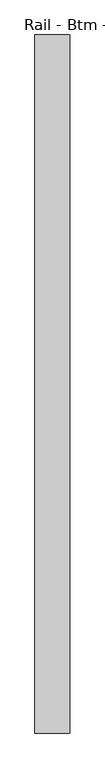
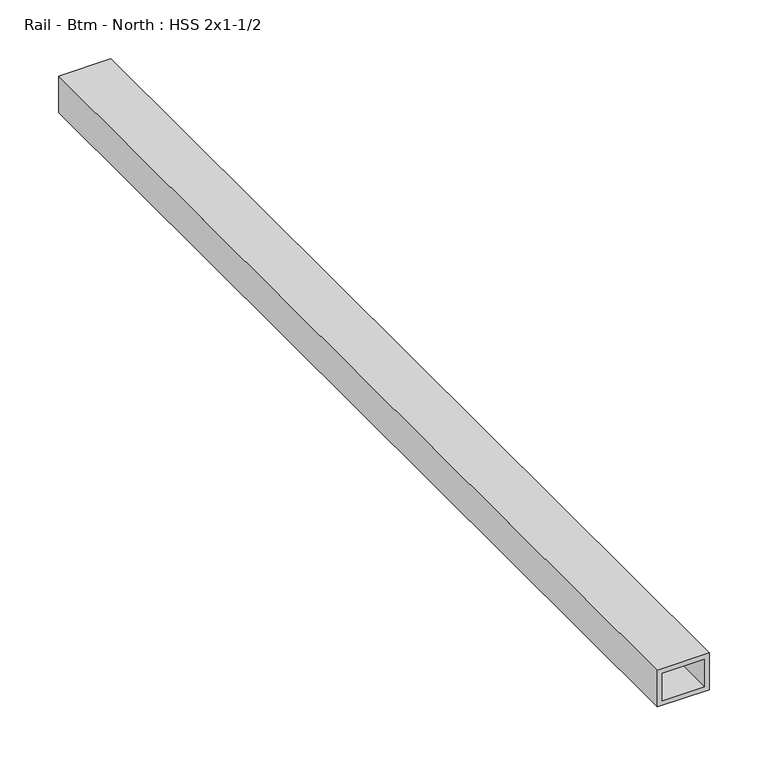
"""IFC4 building model written with IfcOpenShell, lengths in millimetres: proxy geometry, Rail - Btm - North : HSS 2x1-1/2."""

import ifcopenshell
import ifcopenshell.guid

model = None  # the IFC model being written
_history = None  # IfcOwnerHistory: only IFC2X3 demands one
_inside = {}  # id of a spatial element -> (the spatial element, [elements in it])
_under = {}  # id of a project, library or spatial element -> (it, [spatial elements below it])
_declared = {}  # id of a project -> (the project, [libraries it declares])
_typed = {}  # id of a type object -> (the type object, [elements of that type])
_made_of = {}  # id of a material, layer set ... -> (it, [elements and type objects made of it])


def new_model(schema):
    """Start an empty IFC model of exactly this schema.

    Asked for "IFC4X3", IfcOpenShell would pick the latest addendum, in which some entities
    have other attributes; the version numbers below select the first issue.
    IFC2X3 requires an IfcOwnerHistory on every rooted entity: one is made here for all.
    """
    global model, _history
    if schema == "IFC4X3":
        model = ifcopenshell.file(schema_version=(4, 3, 0, 0))
    else:
        model = ifcopenshell.file(schema=schema)
    _inside.clear()
    _under.clear()
    _declared.clear()
    _typed.clear()
    _made_of.clear()
    _history = None
    if model.schema == "IFC2X3":
        org = make("IfcOrganization", Name="unknown")
        user = make(
            "IfcPersonAndOrganization",
            ThePerson=make("IfcPerson", FamilyName="unknown"),
            TheOrganization=org,
        )
        app = make(
            "IfcApplication",
            ApplicationDeveloper=org,
            Version="unknown",
            ApplicationFullName="unknown",
            ApplicationIdentifier="unknown",
        )
        _history = make(
            "IfcOwnerHistory",
            OwningUser=user,
            OwningApplication=app,
            ChangeAction="ADDED",
            CreationDate=0,
        )
    return model


def make(cls, **values):
    """One entity of the class cls with the attributes given. An attribute that is None is left unset."""
    return model.create_entity(
        cls, **{name: value for name, value in values.items() if value is not None}
    )


def rooted(cls, **values):
    """An entity with a GlobalId (a new one), such as an element, a storey or a relation."""
    return make(cls, GlobalId=ifcopenshell.guid.new(), OwnerHistory=_history, **values)


def si_unit(unit_type, name, prefix=None):
    """IfcSIUnit, for example si_unit("LENGTHUNIT", "METRE", prefix="MILLI")."""
    return make("IfcSIUnit", UnitType=unit_type, Prefix=prefix, Name=name)


def assignment(units):
    """IfcUnitAssignment: the units of a project."""
    return None if units is None else make("IfcUnitAssignment", Units=units)


def point(xyz):
    """IfcCartesianPoint."""
    return None if xyz is None else make("IfcCartesianPoint", Coordinates=xyz)


def direction(xyz):
    """IfcDirection."""
    return None if xyz is None else make("IfcDirection", DirectionRatios=xyz)


def frame(location, z_axis=None, x_axis=None):
    """IfcAxis2Placement3D, a coordinate frame: its origin and axes. An axis left out is left unset."""
    return make(
        "IfcAxis2Placement3D",
        Location=point(location),
        Axis=direction(z_axis),
        RefDirection=direction(x_axis),
    )


def origin():
    """The frame at (0, 0, 0) with its axes left unset."""
    return frame((0.0, 0.0, 0.0))


def place(relative_to, where):
    """IfcLocalPlacement: puts the frame where relative to a parent placement (None: the world)."""
    return make(
        "IfcLocalPlacement", PlacementRelTo=relative_to, RelativePlacement=where
    )


def context(
    kind, dimensions, precision=None, world=None, true_north=None, identifier=None
):
    """IfcGeometricRepresentationContext, for example the 3D "Model" context."""
    return make(
        "IfcGeometricRepresentationContext",
        ContextIdentifier=identifier,
        ContextType=kind,
        CoordinateSpaceDimension=dimensions,
        Precision=precision,
        WorldCoordinateSystem=world,
        TrueNorth=true_north,
    )


def project(units=None, contexts=None):
    """IfcProject with its units and contexts."""
    return rooted(
        "IfcProject",
        Name="project",
        RepresentationContexts=contexts,
        UnitsInContext=assignment(units),
    )


def spatial(cls, under=None, at=None, **own):
    """A site, building, storey or space (cls), placed at a placement, below another one or the project."""
    s = rooted(cls, ObjectPlacement=at, **own)
    if under is not None:
        _under.setdefault(under.id(), (under, []))[1].append(s)
    return s


def polyline(points):
    """IfcPolyline through the points."""
    return make("IfcPolyline", Points=[point(p) for p in points])


def outline(outer, holes=None, kind="AREA"):
    """IfcArbitraryClosedProfileDef: a profile drawn as a closed curve; with holes, ...WithVoids."""
    if holes is None:
        return make("IfcArbitraryClosedProfileDef", ProfileType=kind, OuterCurve=outer)
    return make(
        "IfcArbitraryProfileDefWithVoids",
        ProfileType=kind,
        OuterCurve=outer,
        InnerCurves=holes,
    )


def extrude(swept, where, along, depth):
    """IfcExtrudedAreaSolid: the profile swept, set in the frame where, extruded along a direction by depth."""
    return make(
        "IfcExtrudedAreaSolid",
        SweptArea=swept,
        Position=where,
        ExtrudedDirection=direction(along),
        Depth=depth,
    )


def shape(context_of_items, identifier, shape_type, items):
    """IfcShapeRepresentation: the items that make up one representation, for example the "Body"."""
    return make(
        "IfcShapeRepresentation",
        ContextOfItems=context_of_items,
        RepresentationIdentifier=identifier,
        RepresentationType=shape_type,
        Items=items,
    )


def source(mapping_origin, context_of_items, identifier, shape_type, items):
    """IfcRepresentationMap: a shape defined once, which mapped items show again and again."""
    return make(
        "IfcRepresentationMap",
        MappingOrigin=mapping_origin,
        MappedRepresentation=shape(context_of_items, identifier, shape_type, items),
    )


def transform(
    local_origin,
    x_axis=None,
    y_axis=None,
    z_axis=None,
    scale=None,
    scale2=None,
    scale3=None,
    uniform=True,
):
    """IfcCartesianTransformationOperator3D, or its non-uniform kind. x_axis, y_axis, z_axis: its Axis1, 2, 3."""
    if uniform:
        return make(
            "IfcCartesianTransformationOperator3D",
            Axis1=direction(x_axis),
            Axis2=direction(y_axis),
            LocalOrigin=point(local_origin),
            Scale=scale,
            Axis3=direction(z_axis),
        )
    return make(
        "IfcCartesianTransformationOperator3DnonUniform",
        Axis1=direction(x_axis),
        Axis2=direction(y_axis),
        LocalOrigin=point(local_origin),
        Scale=scale,
        Axis3=direction(z_axis),
        Scale2=scale2,
        Scale3=scale3,
    )


def mapped(mapping_source, mapping_target):
    """IfcMappedItem: shows the shape of a source again, moved by a transform."""
    return make(
        "IfcMappedItem", MappingSource=mapping_source, MappingTarget=mapping_target
    )


def made_of(thing, what):
    """Note that an element or type object is made of a material, layer set ...; save() writes the relation."""
    if what is not None:
        _made_of.setdefault(what.id(), (what, []))[1].append(thing)
    return thing


def element(
    cls,
    number,
    at=None,
    inside=None,
    cuts=None,
    type_object=None,
    material=None,
    context=None,
    identifier="Body",
    shape_type=None,
    held_by="IfcProductDefinitionShape",
    body=None,
    shapes=None,
    **own,
):
    """One element of the class cls, such as IfcWall. Its Tag is "e" and its number.

    at: its placement. inside: the storey or other place that contains it. cuts: it is an
    opening in that element (IfcRelVoidsElement). A single representation is given by context,
    identifier, shape_type and body (its items); several are given by shapes. held_by: the class
    of the entity that holds the representations. save() writes the other relations.
    """
    e = rooted(cls, Tag="e%d" % number, ObjectPlacement=at, **own)
    if body is not None:
        shapes = [shape(context, identifier, shape_type, body)]
    if shapes is not None:
        e.Representation = make(held_by, Representations=shapes)
    if inside is not None:
        _inside.setdefault(inside.id(), (inside, []))[1].append(e)
    if cuts is not None:
        rooted(
            "IfcRelVoidsElement", RelatingBuildingElement=cuts, RelatedOpeningElement=e
        )
    if type_object is not None:
        _typed.setdefault(type_object.id(), (type_object, []))[1].append(e)
    return made_of(e, material)


def aggregate(whole, parts):
    """IfcRelAggregates: a whole, such as a stair, and the parts it consists of."""
    return rooted("IfcRelAggregates", RelatingObject=whole, RelatedObjects=parts)


def save(model, path):
    """Write the relations noted so far, then the file.

    IfcRelAggregates (storeys below a building ...), IfcRelContainedInSpatialStructure (elements
    in a storey), IfcRelDefinesByType, IfcRelAssociatesMaterial and IfcRelDeclares: one each for
    every whole, place, type object, material and project.
    """
    for whole, parts in _under.values():
        aggregate(whole, parts)
    for where, things in _inside.values():
        rooted(
            "IfcRelContainedInSpatialStructure",
            RelatedElements=things,
            RelatingStructure=where,
        )
    for kind, things in _typed.values():
        rooted("IfcRelDefinesByType", RelatedObjects=things, RelatingType=kind)
    for what, things in _made_of.values():
        rooted("IfcRelAssociatesMaterial", RelatedObjects=things, RelatingMaterial=what)
    for by, libraries in _declared.values():
        rooted("IfcRelDeclares", RelatingContext=by, RelatedDefinitions=libraries)
    model.write(path)


def rail_btm_north_hss_2x1_1_2_b7e517c1(model_context):
    return source(origin(), model_context, "Body", "SweptSolid", [
        extrude(outline(polyline([(50.8, 587416.6934739), (88.9, 587416.6934739), (88.9, 587365.8934739), (50.8, 587365.8934739), (50.8, 587416.6934739)]), holes=[polyline([(84.1375, 587411.9309739), (55.5625, 587411.9309739), (55.5625, 587370.6559739), (84.1375, 587370.6559739), (84.1375, 587411.9309739)])]), frame((0.0, -532839.3663841, 0.0), z_axis=(0.0, 1.0, 0.0), x_axis=(0.0, 0.0, 1.0)), (0.0, 0.0, 1.0), 1016.0),
    ])


if __name__ == "__main__":
    model = new_model("IFC4")
    model_context = context("Model", 3, world=origin())
    ifc_project = project(units=[si_unit("LENGTHUNIT", "METRE", prefix="MILLI")], contexts=[model_context])
    site = spatial("IfcSite", under=ifc_project)
    building = spatial("IfcBuilding", under=site)
    placement = place(None, origin())
    rail_btm_north_hss_2x1_1_2_shape = rail_btm_north_hss_2x1_1_2_b7e517c1(model_context)
    element("IfcBuildingElementProxy", 1, Name="Rail - Btm - North : HSS 2x1-1/2", ObjectType="Rail - Btm - North : HSS 2x1-1/2", at=placement, inside=building, context=model_context, shape_type="MappedRepresentation", body=[
        mapped(rail_btm_north_hss_2x1_1_2_shape, transform((0.0, 0.0, 0.0), x_axis=(1.0, 0.0, 0.0), y_axis=(0.0, 1.0, 0.0), z_axis=(0.0, 0.0, 1.0))),
    ])
    save(model, "model.ifc")

# Revit data of these elements
# Element 1 (IfcBuildingElementProxy, "Rail - Btm - North : HSS 2x1-1/2")
#   Materials on its faces: "1-1/2\"X2\" GALV. STL HSS TUBING"
# Materials
#   "1-1/2\"X2\" GALV. STL HSS TUBING": class "Generic", colour RGB 211 211 207, transparency 0, Cost = 0
